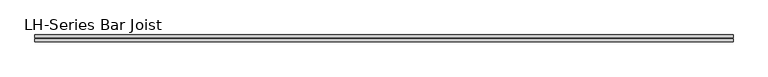
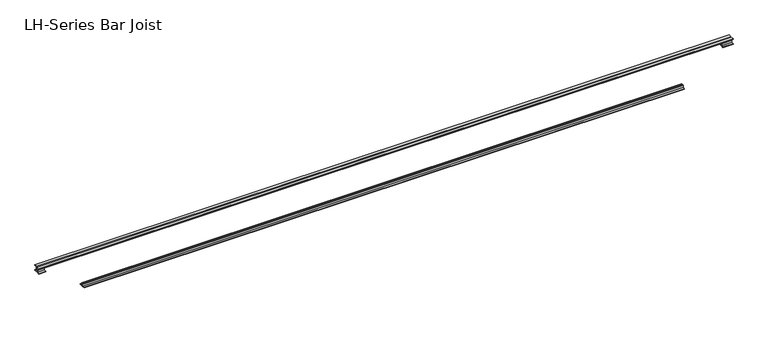
"""IFC4 building model written with IfcOpenShell, lengths in millimetres: beam geometry, LH-Series Bar Joist : GMA_32LH-SP8."""

import ifcopenshell
import ifcopenshell.guid

model = None  # the IFC model being written
_history = None  # IfcOwnerHistory: only IFC2X3 demands one
_inside = {}  # id of a spatial element -> (the spatial element, [elements in it])
_under = {}  # id of a project, library or spatial element -> (it, [spatial elements below it])
_declared = {}  # id of a project -> (the project, [libraries it declares])
_typed = {}  # id of a type object -> (the type object, [elements of that type])
_made_of = {}  # id of a material, layer set ... -> (it, [elements and type objects made of it])


def new_model(schema):
    """Start an empty IFC model of exactly this schema.

    Asked for "IFC4X3", IfcOpenShell would pick the latest addendum, in which some entities
    have other attributes; the version numbers below select the first issue.
    IFC2X3 requires an IfcOwnerHistory on every rooted entity: one is made here for all.
    """
    global model, _history
    if schema == "IFC4X3":
        model = ifcopenshell.file(schema_version=(4, 3, 0, 0))
    else:
        model = ifcopenshell.file(schema=schema)
    _inside.clear()
    _under.clear()
    _declared.clear()
    _typed.clear()
    _made_of.clear()
    _history = None
    if model.schema == "IFC2X3":
        org = make("IfcOrganization", Name="unknown")
        user = make(
            "IfcPersonAndOrganization",
            ThePerson=make("IfcPerson", FamilyName="unknown"),
            TheOrganization=org,
        )
        app = make(
            "IfcApplication",
            ApplicationDeveloper=org,
            Version="unknown",
            ApplicationFullName="unknown",
            ApplicationIdentifier="unknown",
        )
        _history = make(
            "IfcOwnerHistory",
            OwningUser=user,
            OwningApplication=app,
            ChangeAction="ADDED",
            CreationDate=0,
        )
    return model


def make(cls, **values):
    """One entity of the class cls with the attributes given. An attribute that is None is left unset."""
    return model.create_entity(
        cls, **{name: value for name, value in values.items() if value is not None}
    )


def rooted(cls, **values):
    """An entity with a GlobalId (a new one), such as an element, a storey or a relation."""
    return make(cls, GlobalId=ifcopenshell.guid.new(), OwnerHistory=_history, **values)


def si_unit(unit_type, name, prefix=None):
    """IfcSIUnit, for example si_unit("LENGTHUNIT", "METRE", prefix="MILLI")."""
    return make("IfcSIUnit", UnitType=unit_type, Prefix=prefix, Name=name)


def assignment(units):
    """IfcUnitAssignment: the units of a project."""
    return None if units is None else make("IfcUnitAssignment", Units=units)


def point(xyz):
    """IfcCartesianPoint."""
    return None if xyz is None else make("IfcCartesianPoint", Coordinates=xyz)


def direction(xyz):
    """IfcDirection."""
    return None if xyz is None else make("IfcDirection", DirectionRatios=xyz)


def frame(location, z_axis=None, x_axis=None):
    """IfcAxis2Placement3D, a coordinate frame: its origin and axes. An axis left out is left unset."""
    return make(
        "IfcAxis2Placement3D",
        Location=point(location),
        Axis=direction(z_axis),
        RefDirection=direction(x_axis),
    )


def origin():
    """The frame at (0, 0, 0) with its axes left unset."""
    return frame((0.0, 0.0, 0.0))


def place(relative_to, where):
    """IfcLocalPlacement: puts the frame where relative to a parent placement (None: the world)."""
    return make(
        "IfcLocalPlacement", PlacementRelTo=relative_to, RelativePlacement=where
    )


def context(
    kind, dimensions, precision=None, world=None, true_north=None, identifier=None
):
    """IfcGeometricRepresentationContext, for example the 3D "Model" context."""
    return make(
        "IfcGeometricRepresentationContext",
        ContextIdentifier=identifier,
        ContextType=kind,
        CoordinateSpaceDimension=dimensions,
        Precision=precision,
        WorldCoordinateSystem=world,
        TrueNorth=true_north,
    )


def project(units=None, contexts=None):
    """IfcProject with its units and contexts."""
    return rooted(
        "IfcProject",
        Name="project",
        RepresentationContexts=contexts,
        UnitsInContext=assignment(units),
    )


def spatial(cls, under=None, at=None, **own):
    """A site, building, storey or space (cls), placed at a placement, below another one or the project."""
    s = rooted(cls, ObjectPlacement=at, **own)
    if under is not None:
        _under.setdefault(under.id(), (under, []))[1].append(s)
    return s


def polyline(points):
    """IfcPolyline through the points."""
    return make("IfcPolyline", Points=[point(p) for p in points])


def outline(outer, holes=None, kind="AREA"):
    """IfcArbitraryClosedProfileDef: a profile drawn as a closed curve; with holes, ...WithVoids."""
    if holes is None:
        return make("IfcArbitraryClosedProfileDef", ProfileType=kind, OuterCurve=outer)
    return make(
        "IfcArbitraryProfileDefWithVoids",
        ProfileType=kind,
        OuterCurve=outer,
        InnerCurves=holes,
    )


def extrude(swept, where, along, depth):
    """IfcExtrudedAreaSolid: the profile swept, set in the frame where, extruded along a direction by depth."""
    return make(
        "IfcExtrudedAreaSolid",
        SweptArea=swept,
        Position=where,
        ExtrudedDirection=direction(along),
        Depth=depth,
    )


def shape(context_of_items, identifier, shape_type, items):
    """IfcShapeRepresentation: the items that make up one representation, for example the "Body"."""
    return make(
        "IfcShapeRepresentation",
        ContextOfItems=context_of_items,
        RepresentationIdentifier=identifier,
        RepresentationType=shape_type,
        Items=items,
    )


def source(mapping_origin, context_of_items, identifier, shape_type, items):
    """IfcRepresentationMap: a shape defined once, which mapped items show again and again."""
    return make(
        "IfcRepresentationMap",
        MappingOrigin=mapping_origin,
        MappedRepresentation=shape(context_of_items, identifier, shape_type, items),
    )


def transform(
    local_origin,
    x_axis=None,
    y_axis=None,
    z_axis=None,
    scale=None,
    scale2=None,
    scale3=None,
    uniform=True,
):
    """IfcCartesianTransformationOperator3D, or its non-uniform kind. x_axis, y_axis, z_axis: its Axis1, 2, 3."""
    if uniform:
        return make(
            "IfcCartesianTransformationOperator3D",
            Axis1=direction(x_axis),
            Axis2=direction(y_axis),
            LocalOrigin=point(local_origin),
            Scale=scale,
            Axis3=direction(z_axis),
        )
    return make(
        "IfcCartesianTransformationOperator3DnonUniform",
        Axis1=direction(x_axis),
        Axis2=direction(y_axis),
        LocalOrigin=point(local_origin),
        Scale=scale,
        Axis3=direction(z_axis),
        Scale2=scale2,
        Scale3=scale3,
    )


def mapped(mapping_source, mapping_target):
    """IfcMappedItem: shows the shape of a source again, moved by a transform."""
    return make(
        "IfcMappedItem", MappingSource=mapping_source, MappingTarget=mapping_target
    )


def made_of(thing, what):
    """Note that an element or type object is made of a material, layer set ...; save() writes the relation."""
    if what is not None:
        _made_of.setdefault(what.id(), (what, []))[1].append(thing)
    return thing


def element(
    cls,
    number,
    at=None,
    inside=None,
    cuts=None,
    type_object=None,
    material=None,
    context=None,
    identifier="Body",
    shape_type=None,
    held_by="IfcProductDefinitionShape",
    body=None,
    shapes=None,
    **own,
):
    """One element of the class cls, such as IfcWall. Its Tag is "e" and its number.

    at: its placement. inside: the storey or other place that contains it. cuts: it is an
    opening in that element (IfcRelVoidsElement). A single representation is given by context,
    identifier, shape_type and body (its items); several are given by shapes. held_by: the class
    of the entity that holds the representations. save() writes the other relations.
    """
    e = rooted(cls, Tag="e%d" % number, ObjectPlacement=at, **own)
    if body is not None:
        shapes = [shape(context, identifier, shape_type, body)]
    if shapes is not None:
        e.Representation = make(held_by, Representations=shapes)
    if inside is not None:
        _inside.setdefault(inside.id(), (inside, []))[1].append(e)
    if cuts is not None:
        rooted(
            "IfcRelVoidsElement", RelatingBuildingElement=cuts, RelatedOpeningElement=e
        )
    if type_object is not None:
        _typed.setdefault(type_object.id(), (type_object, []))[1].append(e)
    return made_of(e, material)


def aggregate(whole, parts):
    """IfcRelAggregates: a whole, such as a stair, and the parts it consists of."""
    return rooted("IfcRelAggregates", RelatingObject=whole, RelatedObjects=parts)


def save(model, path):
    """Write the relations noted so far, then the file.

    IfcRelAggregates (storeys below a building ...), IfcRelContainedInSpatialStructure (elements
    in a storey), IfcRelDefinesByType, IfcRelAssociatesMaterial and IfcRelDeclares: one each for
    every whole, place, type object, material and project.
    """
    for whole, parts in _under.values():
        aggregate(whole, parts)
    for where, things in _inside.values():
        rooted(
            "IfcRelContainedInSpatialStructure",
            RelatedElements=things,
            RelatingStructure=where,
        )
    for kind, things in _typed.values():
        rooted("IfcRelDefinesByType", RelatedObjects=things, RelatingType=kind)
    for what, things in _made_of.values():
        rooted("IfcRelAssociatesMaterial", RelatedObjects=things, RelatingMaterial=what)
    for by, libraries in _declared.values():
        rooted("IfcRelDeclares", RelatingContext=by, RelatedDefinitions=libraries)
    model.write(path)


def lh_series_bar_joist_ddc9ab2d(model_context):
    return source(origin(), model_context, "Body", "SweptSolid", [
        extrude(outline(polyline([(12.7, 406.4), (76.2, 406.4), (76.2, 393.7), (25.4, 393.7), (25.4, 342.9), (12.7, 342.9), (12.7, 406.4)])), frame((-7750.175, 0.0, 0.0), z_axis=(1.0, 0.0, 0.0), x_axis=(0.0, 1.0, 0.0)), (0.0, 0.0, 1.0), 15576.55),
        extrude(outline(polyline([(-12.7, 406.4), (-12.7, 342.9), (-25.4, 342.9), (-25.4, 393.7), (-76.2, 393.7), (-76.2, 406.4), (-12.7, 406.4)])), frame((-7750.175, 0.0, 0.0), z_axis=(1.0, 0.0, 0.0), x_axis=(0.0, 1.0, 0.0)), (0.0, 0.0, 1.0), 15576.55),
        extrude(outline(polyline([(12.7, -406.4), (12.7, -342.9), (25.4, -342.9), (25.4, -393.7), (76.2, -393.7), (76.2, -406.4), (12.7, -406.4)])), frame((-6734.175, 0.0, 0.0), z_axis=(1.0, 0.0, 0.0), x_axis=(0.0, 1.0, 0.0)), (0.0, 0.0, 1.0), 13468.35),
        extrude(outline(polyline([(-12.7, -406.4), (-76.2, -406.4), (-76.2, -393.7), (-25.4, -393.7), (-25.4, -342.9), (-12.7, -342.9), (-12.7, -406.4)])), frame((-6734.175, 0.0, 0.0), z_axis=(1.0, 0.0, 0.0), x_axis=(0.0, 1.0, 0.0)), (0.0, 0.0, 1.0), 13468.35),
        extrude(outline(polyline([(12.7, 279.4), (12.7, 342.9), (25.4, 342.9), (25.4, 292.1), (76.2, 292.1), (76.2, 279.4), (12.7, 279.4)])), frame((7597.775, 0.0, 0.0), z_axis=(1.0, 0.0, 0.0), x_axis=(0.0, 1.0, 0.0)), (0.0, 0.0, 1.0), 228.6),
        extrude(outline(polyline([(-12.7, 279.4), (-76.2, 279.4), (-76.2, 292.1), (-25.4, 292.1), (-25.4, 342.9), (-12.7, 342.9), (-12.7, 279.4)])), frame((7597.775, 0.0, 0.0), z_axis=(1.0, 0.0, 0.0), x_axis=(0.0, 1.0, 0.0)), (0.0, 0.0, 1.0), 228.6),
        extrude(outline(polyline([(-12.7, 279.4), (-76.2, 279.4), (-76.2, 292.1), (-25.4, 292.1), (-25.4, 342.9), (-12.7, 342.9), (-12.7, 279.4)])), frame((-7750.175, 0.0, 0.0), z_axis=(1.0, 0.0, 0.0), x_axis=(0.0, 1.0, 0.0)), (0.0, 0.0, 1.0), 152.4),
        extrude(outline(polyline([(76.2, 279.4), (12.7, 279.4), (12.7, 342.9), (25.4, 342.9), (25.4, 292.1), (76.2, 292.1), (76.2, 279.4)])), frame((-7750.175, 0.0, 0.0), z_axis=(1.0, 0.0, 0.0), x_axis=(0.0, 1.0, 0.0)), (0.0, 0.0, 1.0), 152.4),
    ])


if __name__ == "__main__":
    model = new_model("IFC4")
    model_context = context("Model", 3, world=origin())
    ifc_project = project(units=[si_unit("LENGTHUNIT", "METRE", prefix="MILLI")], contexts=[model_context])
    site = spatial("IfcSite", under=ifc_project)
    building = spatial("IfcBuilding", under=site)
    placement = place(None, origin())
    lh_series_bar_joist_shape = lh_series_bar_joist_ddc9ab2d(model_context)
    element("IfcBeam", 1, ObjectType="LH-Series Bar Joist : GMA_32LH-SP8", at=placement, inside=building, context=model_context, shape_type="MappedRepresentation", body=[
        mapped(lh_series_bar_joist_shape, transform((0.0, 0.0, 0.0), x_axis=(1.0, 0.0, 0.0), y_axis=(0.0, 1.0, 0.0), z_axis=(0.0, 0.0, 1.0))),
    ])
    save(model, "model.ifc")

# Revit data of these elements
# Type "LH-Series Bar Joist : GMA_32LH-SP8"
#   Assembly Code = "B1010350"
#   Wt = 21
#   Web Thickness = 0' - 1"
#   Variable Panel [instance default] = 5' - 4"
#   Start Offset [instance default] = 0' - 0"
#   Start Extension [instance default] = 0' - 0"
#   Seat Length = 0' - 6"
#   Seat Depth = 0' - 5"
#   IntPanelWidth [instance default] = 5' - 4"
#   IntPanelArrayLength [instance default] = 21' - 4"
#   PanelAreaLength [instance default] = 32' - 0"
#   End Panel = 4' - 0"
#   End Offset [instance default] = 0' - 0"
#   End Extension [instance default] = 0' - 0"
#   Cord Leg = 0' - 2 1/2"
#   Chord Thickness = 0' - 0 1/2"
#   Length [instance default] = 40' - 0"
#   Depth = 2' - 8"
#   Vertical Member Visibility = yes
#   IntPanelArrayNum [instance default] = 4
#   Structural Material = none
# Element 1 (IfcBeam, "LH-Series Bar Joist : GMA_32LH-SP8")
#   Variable Panel = 5' - 5 1/8"
#   IntPanelArrayLength = 32' - 0"
#   PanelAreaLength = 42' - 10 1/4"
#   End Extension = 0' - 3"
#   Length = 50' - 10 1/4"
#   IntPanelArrayNum = 6
